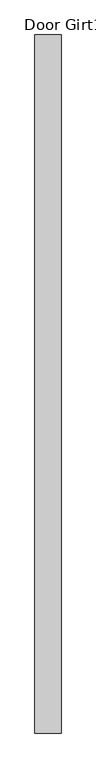
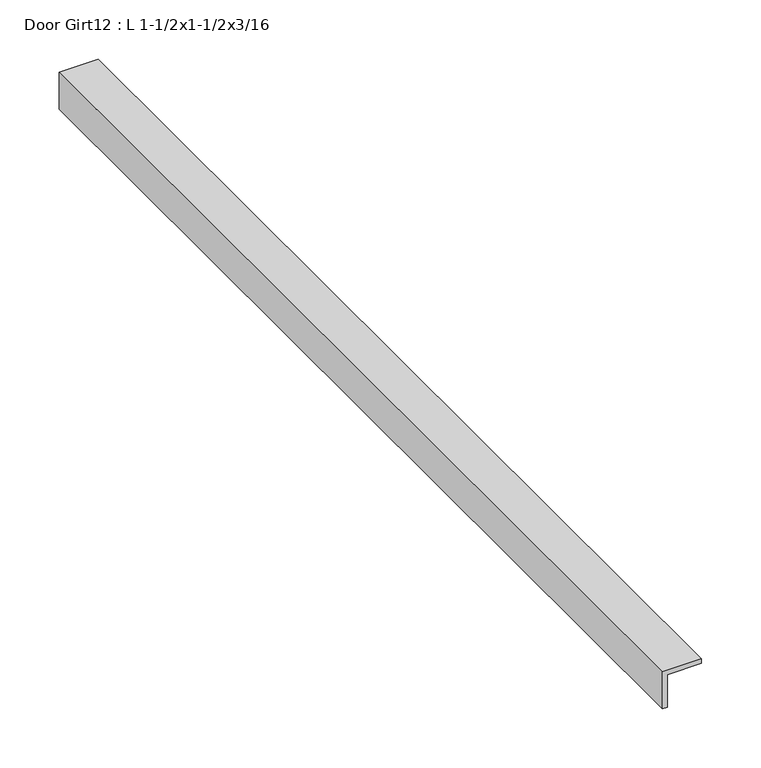
"""IFC4 building model written with IfcOpenShell, lengths in millimetres: proxy geometry, Door Girt12 : L 1-1/2x1-1/2x3/16."""

import ifcopenshell
import ifcopenshell.guid

model = None  # the IFC model being written
_history = None  # IfcOwnerHistory: only IFC2X3 demands one
_inside = {}  # id of a spatial element -> (the spatial element, [elements in it])
_under = {}  # id of a project, library or spatial element -> (it, [spatial elements below it])
_declared = {}  # id of a project -> (the project, [libraries it declares])
_typed = {}  # id of a type object -> (the type object, [elements of that type])
_made_of = {}  # id of a material, layer set ... -> (it, [elements and type objects made of it])


def new_model(schema):
    """Start an empty IFC model of exactly this schema.

    Asked for "IFC4X3", IfcOpenShell would pick the latest addendum, in which some entities
    have other attributes; the version numbers below select the first issue.
    IFC2X3 requires an IfcOwnerHistory on every rooted entity: one is made here for all.
    """
    global model, _history
    if schema == "IFC4X3":
        model = ifcopenshell.file(schema_version=(4, 3, 0, 0))
    else:
        model = ifcopenshell.file(schema=schema)
    _inside.clear()
    _under.clear()
    _declared.clear()
    _typed.clear()
    _made_of.clear()
    _history = None
    if model.schema == "IFC2X3":
        org = make("IfcOrganization", Name="unknown")
        user = make(
            "IfcPersonAndOrganization",
            ThePerson=make("IfcPerson", FamilyName="unknown"),
            TheOrganization=org,
        )
        app = make(
            "IfcApplication",
            ApplicationDeveloper=org,
            Version="unknown",
            ApplicationFullName="unknown",
            ApplicationIdentifier="unknown",
        )
        _history = make(
            "IfcOwnerHistory",
            OwningUser=user,
            OwningApplication=app,
            ChangeAction="ADDED",
            CreationDate=0,
        )
    return model


def make(cls, **values):
    """One entity of the class cls with the attributes given. An attribute that is None is left unset."""
    return model.create_entity(
        cls, **{name: value for name, value in values.items() if value is not None}
    )


def rooted(cls, **values):
    """An entity with a GlobalId (a new one), such as an element, a storey or a relation."""
    return make(cls, GlobalId=ifcopenshell.guid.new(), OwnerHistory=_history, **values)


def si_unit(unit_type, name, prefix=None):
    """IfcSIUnit, for example si_unit("LENGTHUNIT", "METRE", prefix="MILLI")."""
    return make("IfcSIUnit", UnitType=unit_type, Prefix=prefix, Name=name)


def assignment(units):
    """IfcUnitAssignment: the units of a project."""
    return None if units is None else make("IfcUnitAssignment", Units=units)


def point(xyz):
    """IfcCartesianPoint."""
    return None if xyz is None else make("IfcCartesianPoint", Coordinates=xyz)


def direction(xyz):
    """IfcDirection."""
    return None if xyz is None else make("IfcDirection", DirectionRatios=xyz)


def frame(location, z_axis=None, x_axis=None):
    """IfcAxis2Placement3D, a coordinate frame: its origin and axes. An axis left out is left unset."""
    return make(
        "IfcAxis2Placement3D",
        Location=point(location),
        Axis=direction(z_axis),
        RefDirection=direction(x_axis),
    )


def origin():
    """The frame at (0, 0, 0) with its axes left unset."""
    return frame((0.0, 0.0, 0.0))


def place(relative_to, where):
    """IfcLocalPlacement: puts the frame where relative to a parent placement (None: the world)."""
    return make(
        "IfcLocalPlacement", PlacementRelTo=relative_to, RelativePlacement=where
    )


def context(
    kind, dimensions, precision=None, world=None, true_north=None, identifier=None
):
    """IfcGeometricRepresentationContext, for example the 3D "Model" context."""
    return make(
        "IfcGeometricRepresentationContext",
        ContextIdentifier=identifier,
        ContextType=kind,
        CoordinateSpaceDimension=dimensions,
        Precision=precision,
        WorldCoordinateSystem=world,
        TrueNorth=true_north,
    )


def project(units=None, contexts=None):
    """IfcProject with its units and contexts."""
    return rooted(
        "IfcProject",
        Name="project",
        RepresentationContexts=contexts,
        UnitsInContext=assignment(units),
    )


def spatial(cls, under=None, at=None, **own):
    """A site, building, storey or space (cls), placed at a placement, below another one or the project."""
    s = rooted(cls, ObjectPlacement=at, **own)
    if under is not None:
        _under.setdefault(under.id(), (under, []))[1].append(s)
    return s


def polyline(points):
    """IfcPolyline through the points."""
    return make("IfcPolyline", Points=[point(p) for p in points])


def outline(outer, holes=None, kind="AREA"):
    """IfcArbitraryClosedProfileDef: a profile drawn as a closed curve; with holes, ...WithVoids."""
    if holes is None:
        return make("IfcArbitraryClosedProfileDef", ProfileType=kind, OuterCurve=outer)
    return make(
        "IfcArbitraryProfileDefWithVoids",
        ProfileType=kind,
        OuterCurve=outer,
        InnerCurves=holes,
    )


def extrude(swept, where, along, depth):
    """IfcExtrudedAreaSolid: the profile swept, set in the frame where, extruded along a direction by depth."""
    return make(
        "IfcExtrudedAreaSolid",
        SweptArea=swept,
        Position=where,
        ExtrudedDirection=direction(along),
        Depth=depth,
    )


def shape(context_of_items, identifier, shape_type, items):
    """IfcShapeRepresentation: the items that make up one representation, for example the "Body"."""
    return make(
        "IfcShapeRepresentation",
        ContextOfItems=context_of_items,
        RepresentationIdentifier=identifier,
        RepresentationType=shape_type,
        Items=items,
    )


def source(mapping_origin, context_of_items, identifier, shape_type, items):
    """IfcRepresentationMap: a shape defined once, which mapped items show again and again."""
    return make(
        "IfcRepresentationMap",
        MappingOrigin=mapping_origin,
        MappedRepresentation=shape(context_of_items, identifier, shape_type, items),
    )


def transform(
    local_origin,
    x_axis=None,
    y_axis=None,
    z_axis=None,
    scale=None,
    scale2=None,
    scale3=None,
    uniform=True,
):
    """IfcCartesianTransformationOperator3D, or its non-uniform kind. x_axis, y_axis, z_axis: its Axis1, 2, 3."""
    if uniform:
        return make(
            "IfcCartesianTransformationOperator3D",
            Axis1=direction(x_axis),
            Axis2=direction(y_axis),
            LocalOrigin=point(local_origin),
            Scale=scale,
            Axis3=direction(z_axis),
        )
    return make(
        "IfcCartesianTransformationOperator3DnonUniform",
        Axis1=direction(x_axis),
        Axis2=direction(y_axis),
        LocalOrigin=point(local_origin),
        Scale=scale,
        Axis3=direction(z_axis),
        Scale2=scale2,
        Scale3=scale3,
    )


def mapped(mapping_source, mapping_target):
    """IfcMappedItem: shows the shape of a source again, moved by a transform."""
    return make(
        "IfcMappedItem", MappingSource=mapping_source, MappingTarget=mapping_target
    )


def made_of(thing, what):
    """Note that an element or type object is made of a material, layer set ...; save() writes the relation."""
    if what is not None:
        _made_of.setdefault(what.id(), (what, []))[1].append(thing)
    return thing


def element(
    cls,
    number,
    at=None,
    inside=None,
    cuts=None,
    type_object=None,
    material=None,
    context=None,
    identifier="Body",
    shape_type=None,
    held_by="IfcProductDefinitionShape",
    body=None,
    shapes=None,
    **own,
):
    """One element of the class cls, such as IfcWall. Its Tag is "e" and its number.

    at: its placement. inside: the storey or other place that contains it. cuts: it is an
    opening in that element (IfcRelVoidsElement). A single representation is given by context,
    identifier, shape_type and body (its items); several are given by shapes. held_by: the class
    of the entity that holds the representations. save() writes the other relations.
    """
    e = rooted(cls, Tag="e%d" % number, ObjectPlacement=at, **own)
    if body is not None:
        shapes = [shape(context, identifier, shape_type, body)]
    if shapes is not None:
        e.Representation = make(held_by, Representations=shapes)
    if inside is not None:
        _inside.setdefault(inside.id(), (inside, []))[1].append(e)
    if cuts is not None:
        rooted(
            "IfcRelVoidsElement", RelatingBuildingElement=cuts, RelatedOpeningElement=e
        )
    if type_object is not None:
        _typed.setdefault(type_object.id(), (type_object, []))[1].append(e)
    return made_of(e, material)


def aggregate(whole, parts):
    """IfcRelAggregates: a whole, such as a stair, and the parts it consists of."""
    return rooted("IfcRelAggregates", RelatingObject=whole, RelatedObjects=parts)


def save(model, path):
    """Write the relations noted so far, then the file.

    IfcRelAggregates (storeys below a building ...), IfcRelContainedInSpatialStructure (elements
    in a storey), IfcRelDefinesByType, IfcRelAssociatesMaterial and IfcRelDeclares: one each for
    every whole, place, type object, material and project.
    """
    for whole, parts in _under.values():
        aggregate(whole, parts)
    for where, things in _inside.values():
        rooted(
            "IfcRelContainedInSpatialStructure",
            RelatedElements=things,
            RelatingStructure=where,
        )
    for kind, things in _typed.values():
        rooted("IfcRelDefinesByType", RelatedObjects=things, RelatingType=kind)
    for what, things in _made_of.values():
        rooted("IfcRelAssociatesMaterial", RelatedObjects=things, RelatingMaterial=what)
    for by, libraries in _declared.values():
        rooted("IfcRelDeclares", RelatingContext=by, RelatedDefinitions=libraries)
    model.write(path)


def door_girt12_l_1_1_2x1_1_2x3_16_372e9288(model_context):
    return source(origin(), model_context, "Body", "SweptSolid", [
        extrude(outline(polyline([(1625.6, 587403.9934739), (1625.6, 587365.8934739), (1587.5, 587365.8934739), (1587.5, 587370.6559739), (1620.8375, 587370.6559739), (1620.8375, 587403.9934739), (1625.6, 587403.9934739)])), frame((0.0, -536263.6038841, 0.0), z_axis=(0.0, 1.0, 0.0), x_axis=(0.0, 0.0, 1.0)), (0.0, 0.0, 1.0), 1017.5875),
    ])


if __name__ == "__main__":
    model = new_model("IFC4")
    model_context = context("Model", 3, world=origin())
    ifc_project = project(units=[si_unit("LENGTHUNIT", "METRE", prefix="MILLI")], contexts=[model_context])
    site = spatial("IfcSite", under=ifc_project)
    building = spatial("IfcBuilding", under=site)
    placement = place(None, origin())
    door_girt12_l_1_1_2x1_1_2x3_16_shape = door_girt12_l_1_1_2x1_1_2x3_16_372e9288(model_context)
    element("IfcBuildingElementProxy", 1, Name="Door Girt12 : L 1-1/2x1-1/2x3/16", ObjectType="Door Girt12 : L 1-1/2x1-1/2x3/16", at=placement, inside=building, context=model_context, shape_type="MappedRepresentation", body=[
        mapped(door_girt12_l_1_1_2x1_1_2x3_16_shape, transform((0.0, 0.0, 0.0), x_axis=(1.0, 0.0, 0.0), y_axis=(0.0, 1.0, 0.0), z_axis=(0.0, 0.0, 1.0))),
    ])
    save(model, "model.ifc")

# Revit data of these elements
# Element 1 (IfcBuildingElementProxy, "Door Girt12 : L 1-1/2x1-1/2x3/16")
#   Materials on its faces: "1-1/2\"X1-1/2\" GALV. STL L"
# Materials
#   "1-1/2\"X1-1/2\" GALV. STL L": class "Generic", colour RGB 211 211 207, transparency 0, Cost = 0
